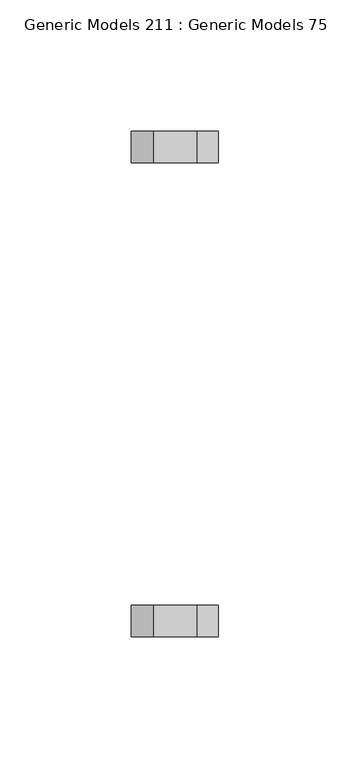
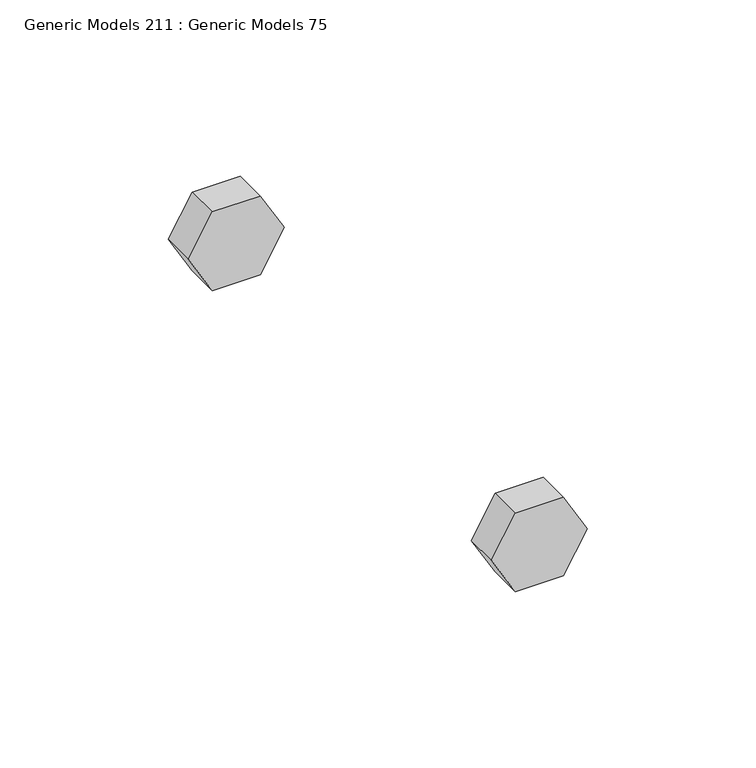
"""IFC4 building model written with IfcOpenShell, lengths in millimetres: proxy geometry, Generic Models 211 : Generic Models 75."""

from ifc_helpers import new_model, si_unit, frame, origin, place, context, project, spatial, polyline, outline, extrude, source, transform, mapped, element, save


def generic_models_211_generic_models_75_f9ca25a0(model_context):
    return source(origin(), model_context, "Body", "SweptSolid", [
        extrude(outline(polyline([(271733.9625, 31978.2851858), (271733.9625, 31994.7829698), (271748.25, 32003.0318618), (271762.5375, 31994.7829698), (271762.5375, 31978.2851858), (271748.25, 31970.0362939), (271733.9625, 31978.2851858)])), frame((0.0, 30678.2969112, 0.0), z_axis=(0.0, 1.0, 0.0), x_axis=(0.0, 0.0, 1.0)), (0.0, 0.0, 1.0), 11.90625),
        extrude(outline(polyline([(271733.9625, 31978.2851858), (271733.9625, 31994.7829698), (271748.25, 32003.0318618), (271762.5375, 31994.7829698), (271762.5375, 31978.2851858), (271748.25, 31970.0362939), (271733.9625, 31978.2851858)])), frame((0.0, 30858.4781612, 0.0), z_axis=(0.0, 1.0, 0.0), x_axis=(0.0, 0.0, 1.0)), (0.0, 0.0, 1.0), 11.90625),
    ])


if __name__ == "__main__":
    model = new_model("IFC4")
    model_context = context("Model", 3, world=origin())
    ifc_project = project(units=[si_unit("LENGTHUNIT", "METRE", prefix="MILLI")], contexts=[model_context])
    site = spatial("IfcSite", under=ifc_project)
    building = spatial("IfcBuilding", under=site)
    placement = place(None, origin())
    generic_models_211_generic_models_75_shape = generic_models_211_generic_models_75_f9ca25a0(model_context)
    element("IfcBuildingElementProxy", 1, Name="Generic Models 211 : Generic Models 75", ObjectType="Generic Models 211 : Generic Models 75", at=placement, inside=building, context=model_context, shape_type="MappedRepresentation", body=[
        mapped(generic_models_211_generic_models_75_shape, transform((0.0, 0.0, 0.0), x_axis=(1.0, 0.0, 0.0), y_axis=(0.0, 1.0, 0.0), z_axis=(0.0, 0.0, 1.0))),
    ])
    save(model, "model.ifc")

# Revit data of these elements
# Element 1 (IfcBuildingElementProxy, "Generic Models 211 : Generic Models 75")
#   Materials on its faces: "3/4\" GALV. THRU BOLTS"
# Materials
#   "3/4\" GALV. THRU BOLTS": class "Generic", colour RGB 105 69 171, transparency 0, Cost = 0
